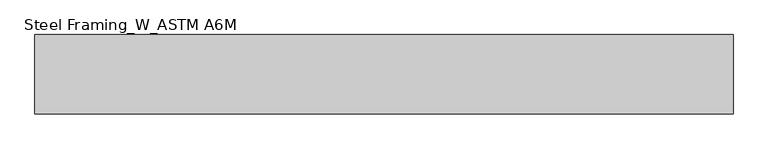
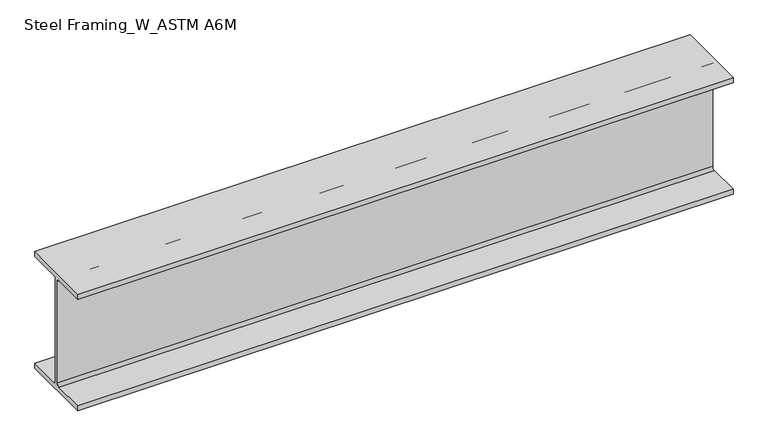
"""IFC4 building model written with IfcOpenShell, lengths in millimetres: beam geometry, Steel Framing_W_ASTM A6M : H_SB_AR_S02_W460x128_B1."""

from ifc_helpers import new_model, si_unit, point, frame, frame_2d, origin, place, context, project, spatial, polyline, circle_curve, trimmed, segment, composite_curve, outline, extrude, source, transform, mapped, element, save


def steel_framing_w_astm_a6m_6e95f1e3(model_context):
    return source(origin(), model_context, "Body", "SweptSolid", [
        extrude(outline(composite_curve([segment(polyline([(141.0, -213.9), (141.0, -233.5), (-141.0, -233.5), (-141.0, -213.9), (-16.2, -213.9)]), True, "CONTINUOUS"), segment(trimmed(circle_curve(frame_2d((-16.2, -203.8)), 10.1), [point((-16.2, -213.9))], [point((-6.1, -203.8))], True, "CARTESIAN"), True, "CONTINUOUS"), segment(polyline([(-6.1, -203.8), (-6.1, 203.8)]), True, "CONTINUOUS"), segment(trimmed(circle_curve(frame_2d((-16.2, 203.8)), 10.1), [point((-6.1, 203.8))], [point((-16.2, 213.9))], True, "CARTESIAN"), True, "CONTINUOUS"), segment(polyline([(-16.2, 213.9), (-141.0, 213.9), (-141.0, 233.5), (141.0, 233.5), (141.0, 213.9), (16.2, 213.9)]), True, "CONTINUOUS"), segment(trimmed(circle_curve(frame_2d((16.2, 203.8)), 10.1), [point((16.2, 213.9))], [point((6.1, 203.8))], True, "CARTESIAN"), True, "CONTINUOUS"), segment(polyline([(6.1, 203.8), (6.1, -203.8)]), True, "CONTINUOUS"), segment(trimmed(circle_curve(frame_2d((16.2, -203.8)), 10.1), [point((6.1, -203.8))], [point((16.2, -213.9))], True, "CARTESIAN"), True, "CONTINUOUS"), segment(polyline([(16.2, -213.9), (141.0, -213.9)]), True, "CONTINUOUS")], self_intersect=False)), frame((-1133.3, 0.0, 0.0), z_axis=(1.0, 0.0, 0.0), x_axis=(0.0, 1.0, 0.0)), (0.0, 0.0, 1.0), 2479.6),
    ])


if __name__ == "__main__":
    model = new_model("IFC4")
    model_context = context("Model", 3, world=origin())
    ifc_project = project(units=[si_unit("LENGTHUNIT", "METRE", prefix="MILLI")], contexts=[model_context])
    site = spatial("IfcSite", under=ifc_project)
    building = spatial("IfcBuilding", under=site)
    placement = place(None, origin())
    steel_framing_w_astm_a6m_shape = steel_framing_w_astm_a6m_6e95f1e3(model_context)
    element("IfcBeam", 1, ObjectType="Steel Framing_W_ASTM A6M : H_SB_AR_S02_W460x128_B1", at=placement, inside=building, context=model_context, shape_type="MappedRepresentation", body=[
        mapped(steel_framing_w_astm_a6m_shape, transform((0.0, 0.0, 0.0), x_axis=(1.0, 0.0, 0.0), y_axis=(0.0, 1.0, 0.0), z_axis=(0.0, 0.0, 1.0))),
    ])
    save(model, "model.ifc")

# Revit data of these elements
# Type "Steel Framing_W_ASTM A6M : H_SB_AR_S02_W460x128_B1"
#   Section Name Key = "W18x86"
#   Width = 28.2 cm
#   Web Thickness = 1.22 cm
#   Web Fillet = 1.01 cm
#   Warping Constant = 3650000.0 cm⁶
#   Torsional Moment of Inertia = 171.00 cm⁴
#   Section Area = 163.0 cm²
#   Plastic Modulus weak axis = 793.0 cm³
#   Plastic Modulus strong axis = 3050.0 cm³
#   Perimeter = 2.02 m²/m
#   Nominal Weight = 128.00 kgf/m
#   Moment of Inertia weak axis = 7280.00 cm⁴
#   Moment of Inertia strong axis = 63700.00 cm⁴
#   Height = 46.7 cm
#   Flange Thickness = 1.96 cm
#   Elastic Modulus weak axis = 518.0 cm³
#   Elastic Modulus strong axis = 2720.0 cm³
#   Centroid Vertical = 23.35 cm
#   Centroid Horizontal = 14.1 cm
#   Length [instance default] = 1500 mm
#   Structural Material [instance default] = Steel, 45-345
#   Bolt Spacing = 0
#   Assembly Code = ""
# Element 1 (IfcBeam, "Steel Framing_W_ASTM A6M : H_SB_AR_S02_W460x128_B1")
#   Materials on its faces: "Steel, 45-345"
# Materials
#   "Steel, 45-345": class "Metal", colour RGB 189 187 185, transparency 0, Description = "Steel 345 MPa", Cost = 0
